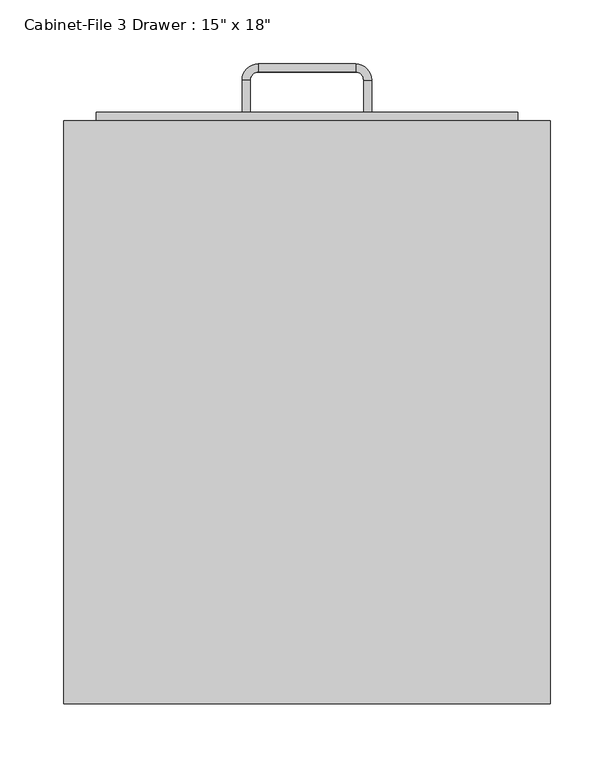
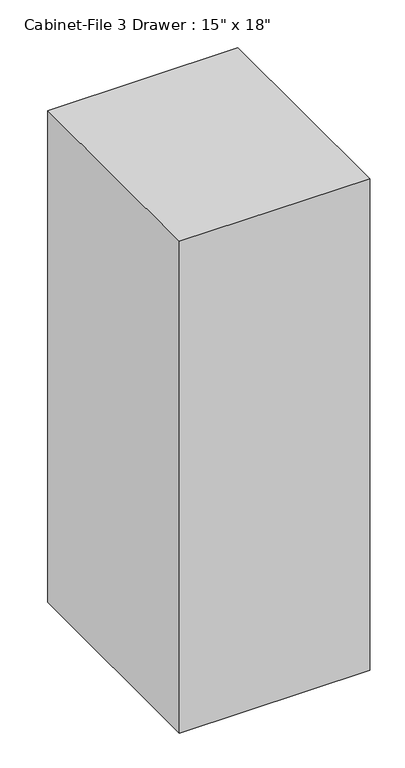
"""IFC4 building model written with IfcOpenShell, lengths in millimetres: furniture geometry."""

from ifc_helpers import new_model, si_unit, frame, origin, origin_with_axes, place, context, project, spatial, polyline, circle_curve, outline, extrude, source, transform, mapped, element, save
from ifc_brep_helpers import plane_surface, cylinder_surface, revolved_surface, advanced_brep


def furniture_48aa8ab9(model_context):
    return source(origin(), model_context, "Body", "SolidModel", [
        extrude(outline(polyline([(62.603553, -86.4656999), (-318.396447, -86.4656999), (-318.396447, 370.7343001), (62.603553, 370.7343001), (62.603553, -86.4656999)])), origin_with_axes(), (0.0, 0.0, 1.0), 1041.4),
        extrude(outline(polyline([(37.203553, 377.0843001), (37.203553, 370.7343001), (-292.996447, 370.7343001), (-292.996447, 377.0843001), (37.203553, 377.0843001)])), frame((0.0, 0.0, 736.6), z_axis=(0.0, 0.0, 1.0), x_axis=(1.0, 0.0, 0.0)), (0.0, 0.0, 1.0), 279.4),
        extrude(outline(polyline([(37.203553, 377.0843001), (37.203553, 370.7343001), (-292.996447, 370.7343001), (-292.996447, 377.0843001), (37.203553, 377.0843001)])), frame((0.0, 0.0, 431.8), z_axis=(0.0, 0.0, 1.0), x_axis=(1.0, 0.0, 0.0)), (0.0, 0.0, 1.0), 279.4),
        extrude(outline(polyline([(37.203553, 377.0843001), (37.203553, 370.7343001), (-292.996447, 370.7343001), (-292.996447, 377.0843001), (37.203553, 377.0843001)])), frame((0.0, 0.0, 127.0), z_axis=(0.0, 0.0, 1.0), x_axis=(1.0, 0.0, 0.0)), (0.0, 0.0, 1.0), 279.4),
        advanced_brep(
        [(-172.346447, 377.0843001, 203.2), (-172.346447, 377.0843001, 215.9), (-178.696447, 377.0843001, 215.9), (-178.696447, 377.0843001, 203.2), (-178.696447, 402.4843001, 203.2), (-172.346447, 402.4843001, 203.2), (-178.696447, 402.4843001, 215.9), (-172.346447, 402.4843001, 215.9), (-165.996447, 415.1843001, 203.2), (-165.996447, 408.8343001, 203.2), (-165.996447, 415.1843001, 215.9), (-165.996447, 408.8343001, 215.9), (-89.796447, 415.1843001, 203.2), (-89.796447, 408.8343001, 203.2), (-89.796447, 415.1843001, 215.9), (-89.796447, 408.8343001, 215.9), (-77.096447, 402.4843001, 203.2), (-83.446447, 402.4843001, 203.2), (-77.096447, 402.4843001, 215.9), (-83.446447, 402.4843001, 215.9), (-83.446447, 377.0843001, 203.2), (-77.096447, 377.0843001, 203.2), (-77.096447, 377.0843001, 215.9), (-83.446447, 377.0843001, 215.9)],
        [
            (0, 1),
            (1, 2),
            (2, 3),
            (3, 0),
            (3, 4),
            (4, 5),
            (5, 0),
            (2, 6),
            (6, 4),
            (1, 7),
            (7, 6),
            (5, 7),
            (8, 9),
            (9, 5, circle_curve(frame((-165.996447, 402.4843001, 203.2), z_axis=(0.0, 0.0, 1.0), x_axis=(-1.0, 0.0, 0.0)), 6.35)),
            (4, 8, circle_curve(frame((-165.996447, 402.4843001, 203.2), z_axis=(0.0, 0.0, -1.0), x_axis=(-1.0, 0.0, 0.0)), 12.7)),
            (10, 8),
            (6, 10, circle_curve(frame((-165.996447, 402.4843001, 215.9), z_axis=(0.0, 0.0, -1.0), x_axis=(-1.0, 0.0, 0.0)), 12.7)),
            (11, 10),
            (7, 11, circle_curve(frame((-165.996447, 402.4843001, 215.9), z_axis=(0.0, 0.0, -1.0), x_axis=(-1.0, 0.0, 0.0)), 6.35)),
            (9, 11),
            (8, 12),
            (12, 13),
            (13, 9),
            (10, 14),
            (14, 12),
            (11, 15),
            (15, 14),
            (13, 15),
            (16, 17),
            (17, 13, circle_curve(frame((-89.796447, 402.4843001, 203.2), z_axis=(0.0, 0.0, 1.0), x_axis=(0.0, 1.0, 0.0)), 6.35)),
            (12, 16, circle_curve(frame((-89.796447, 402.4843001, 203.2), z_axis=(0.0, 0.0, -1.0), x_axis=(0.0, 1.0, 0.0)), 12.7)),
            (18, 16),
            (14, 18, circle_curve(frame((-89.796447, 402.4843001, 215.9), z_axis=(0.0, 0.0, -1.0), x_axis=(0.0, 1.0, 0.0)), 12.7)),
            (19, 18),
            (15, 19, circle_curve(frame((-89.796447, 402.4843001, 215.9), z_axis=(0.0, 0.0, -1.0), x_axis=(0.0, 1.0, 0.0)), 6.35)),
            (17, 19),
            (20, 21),
            (21, 22),
            (22, 23),
            (23, 20),
            (16, 21),
            (20, 17),
            (18, 22),
            (19, 23),
        ],
        [
            plane_surface(frame((-978.8216451, 377.0843001, 0.0), z_axis=(0.0, -1.0, 0.0), x_axis=(0.0, 0.0, -1.0))),
            plane_surface(frame((-172.346447, 377.0843001, 203.2), z_axis=(0.0, 0.0, -1.0), x_axis=(0.0, 1.0, 0.0))),
            plane_surface(frame((-178.696447, 377.0843001, 203.2), z_axis=(-1.0, 0.0, 0.0), x_axis=(0.0, 1.0, 0.0))),
            plane_surface(frame((-178.696447, 377.0843001, 215.9), z_axis=(0.0, 0.0, 1.0), x_axis=(0.0, 1.0, 0.0))),
            plane_surface(frame((-172.346447, 377.0843001, 215.9), z_axis=(1.0, 0.0, 0.0), x_axis=(0.0, 1.0, 0.0))),
            plane_surface(frame((-165.996447, 402.4843001, 203.2), z_axis=(0.0, 0.0, -1.0), x_axis=(-1.0, 0.0, 0.0))),
            cylinder_surface(frame((-165.996447, 402.4843001, 0.0), z_axis=(0.0, 0.0, 1.0), x_axis=(-1.0, 0.0, 0.0)), 12.7),
            plane_surface(frame((-165.996447, 402.4843001, 215.9), z_axis=(0.0, 0.0, 1.0), x_axis=(-1.0, 0.0, 0.0))),
            revolved_surface(polyline([(-172.34644699999998, 402.4843001, 215.9), (-172.34644699999998, 402.4843001, 203.2)]), (-165.996447, 402.4843001, 0.0), (0.0, 0.0, 1.0)),
            plane_surface(frame((-165.996447, 408.8343001, 203.2), z_axis=(0.0, 0.0, -1.0), x_axis=(1.0, 0.0, 0.0))),
            plane_surface(frame((-165.996447, 415.1843001, 203.2), z_axis=(0.0, 1.0, 0.0), x_axis=(1.0, 0.0, 0.0))),
            plane_surface(frame((-165.996447, 415.1843001, 215.9), z_axis=(0.0, 0.0, 1.0), x_axis=(1.0, 0.0, 0.0))),
            plane_surface(frame((-165.996447, 408.8343001, 215.9), z_axis=(0.0, -1.0, 0.0), x_axis=(1.0, 0.0, 0.0))),
            plane_surface(frame((-89.796447, 402.4843001, 203.2), z_axis=(0.0, 0.0, -1.0), x_axis=(0.0, 1.0, 0.0))),
            cylinder_surface(frame((-89.796447, 402.4843001, 0.0), z_axis=(0.0, 0.0, 1.0), x_axis=(0.0, 1.0, 0.0)), 12.7),
            plane_surface(frame((-89.796447, 402.4843001, 215.9), z_axis=(0.0, 0.0, 1.0), x_axis=(0.0, 1.0, 0.0))),
            revolved_surface(polyline([(-89.796447, 408.8343001, 215.9), (-89.796447, 408.8343001, 203.2)]), (-89.796447, 402.4843001, 0.0), (0.0, 0.0, 1.0)),
            plane_surface(frame((-877.2216451, 377.0843001, 0.0), z_axis=(0.0, -1.0, 0.0), x_axis=(0.0, 0.0, 1.0))),
            plane_surface(frame((-83.446447, 402.4843001, 203.2), z_axis=(0.0, 0.0, -1.0), x_axis=(0.0, -1.0, 0.0))),
            plane_surface(frame((-77.096447, 402.4843001, 203.2), z_axis=(1.0, 0.0, 0.0), x_axis=(0.0, -1.0, 0.0))),
            plane_surface(frame((-77.096447, 402.4843001, 215.9), z_axis=(0.0, 0.0, 1.0), x_axis=(0.0, -1.0, 0.0))),
            plane_surface(frame((-83.446447, 402.4843001, 215.9), z_axis=(-1.0, 0.0, 0.0), x_axis=(0.0, -1.0, 0.0))),
        ],
        [
            (0, [[1, 2, 3, 4]]),
            (1, [[5, 6, 7, -4]]),
            (2, [[8, 9, -5, -3]]),
            (3, [[10, 11, -8, -2]]),
            (4, [[-7, 12, -10, -1]]),
            (5, [[13, 14, -6, 15]]),
            (6, [[16, -15, -9, 17]]),
            (7, [[18, -17, -11, 19]]),
            (8, [[20, -19, -12, -14]]),
            (9, [[21, 22, 23, -13]]),
            (10, [[24, 25, -21, -16]]),
            (11, [[26, 27, -24, -18]]),
            (12, [[-23, 28, -26, -20]]),
            (13, [[29, 30, -22, 31]]),
            (14, [[32, -31, -25, 33]]),
            (15, [[34, -33, -27, 35]]),
            (16, [[36, -35, -28, -30]]),
            (17, [[37, 38, 39, 40]]),
            (18, [[41, -37, 42, -29]]),
            (19, [[43, -38, -41, -32]]),
            (20, [[44, -39, -43, -34]]),
            (21, [[-42, -40, -44, -36]]),
        ],
    ),
        advanced_brep(
        [(-172.346447, 377.0843001, 482.6), (-172.346447, 377.0843001, 495.3), (-178.696447, 377.0843001, 495.3), (-178.696447, 377.0843001, 482.6), (-178.696447, 402.4843001, 482.6), (-172.346447, 402.4843001, 482.6), (-178.696447, 402.4843001, 495.3), (-172.346447, 402.4843001, 495.3), (-165.996447, 415.1843001, 482.6), (-165.996447, 408.8343001, 482.6), (-165.996447, 415.1843001, 495.3), (-165.996447, 408.8343001, 495.3), (-89.796447, 415.1843001, 482.6), (-89.796447, 408.8343001, 482.6), (-89.796447, 415.1843001, 495.3), (-89.796447, 408.8343001, 495.3), (-77.096447, 402.4843001, 482.6), (-83.446447, 402.4843001, 482.6), (-77.096447, 402.4843001, 495.3), (-83.446447, 402.4843001, 495.3), (-83.446447, 377.0843001, 482.6), (-77.096447, 377.0843001, 482.6), (-77.096447, 377.0843001, 495.3), (-83.446447, 377.0843001, 495.3)],
        [
            (0, 1),
            (1, 2),
            (2, 3),
            (3, 0),
            (3, 4),
            (4, 5),
            (5, 0),
            (2, 6),
            (6, 4),
            (1, 7),
            (7, 6),
            (5, 7),
            (8, 9),
            (9, 5, circle_curve(frame((-165.996447, 402.4843001, 482.6), z_axis=(0.0, 0.0, 1.0), x_axis=(-1.0, 0.0, 0.0)), 6.35)),
            (4, 8, circle_curve(frame((-165.996447, 402.4843001, 482.6), z_axis=(0.0, 0.0, -1.0), x_axis=(-1.0, 0.0, 0.0)), 12.7)),
            (10, 8),
            (6, 10, circle_curve(frame((-165.996447, 402.4843001, 495.3), z_axis=(0.0, 0.0, -1.0), x_axis=(-1.0, 0.0, 0.0)), 12.7)),
            (11, 10),
            (7, 11, circle_curve(frame((-165.996447, 402.4843001, 495.3), z_axis=(0.0, 0.0, -1.0), x_axis=(-1.0, 0.0, 0.0)), 6.35)),
            (9, 11),
            (8, 12),
            (12, 13),
            (13, 9),
            (10, 14),
            (14, 12),
            (11, 15),
            (15, 14),
            (13, 15),
            (16, 17),
            (17, 13, circle_curve(frame((-89.796447, 402.4843001, 482.6), z_axis=(0.0, 0.0, 1.0), x_axis=(0.0, 1.0, 0.0)), 6.35)),
            (12, 16, circle_curve(frame((-89.796447, 402.4843001, 482.6), z_axis=(0.0, 0.0, -1.0), x_axis=(0.0, 1.0, 0.0)), 12.7)),
            (18, 16),
            (14, 18, circle_curve(frame((-89.796447, 402.4843001, 495.3), z_axis=(0.0, 0.0, -1.0), x_axis=(0.0, 1.0, 0.0)), 12.7)),
            (19, 18),
            (15, 19, circle_curve(frame((-89.796447, 402.4843001, 495.3), z_axis=(0.0, 0.0, -1.0), x_axis=(0.0, 1.0, 0.0)), 6.35)),
            (17, 19),
            (20, 21),
            (21, 22),
            (22, 23),
            (23, 20),
            (16, 21),
            (20, 17),
            (18, 22),
            (19, 23),
        ],
        [
            plane_surface(frame((-978.8216451, 377.0843001, 0.0), z_axis=(0.0, -1.0, 0.0), x_axis=(0.0, 0.0, -1.0))),
            plane_surface(frame((-172.346447, 377.0843001, 482.6), z_axis=(0.0, 0.0, -1.0), x_axis=(0.0, 1.0, 0.0))),
            plane_surface(frame((-178.696447, 377.0843001, 482.6), z_axis=(-1.0, 0.0, 0.0), x_axis=(0.0, 1.0, 0.0))),
            plane_surface(frame((-178.696447, 377.0843001, 495.3), z_axis=(0.0, 0.0, 1.0), x_axis=(0.0, 1.0, 0.0))),
            plane_surface(frame((-172.346447, 377.0843001, 495.3), z_axis=(1.0, 0.0, 0.0), x_axis=(0.0, 1.0, 0.0))),
            plane_surface(frame((-165.996447, 402.4843001, 482.6), z_axis=(0.0, 0.0, -1.0), x_axis=(-1.0, 0.0, 0.0))),
            cylinder_surface(frame((-165.996447, 402.4843001, 0.0), z_axis=(0.0, 0.0, 1.0), x_axis=(-1.0, 0.0, 0.0)), 12.7),
            plane_surface(frame((-165.996447, 402.4843001, 495.3), z_axis=(0.0, 0.0, 1.0), x_axis=(-1.0, 0.0, 0.0))),
            revolved_surface(polyline([(-172.34644699999998, 402.4843001, 495.3), (-172.34644699999998, 402.4843001, 482.6)]), (-165.996447, 402.4843001, 0.0), (0.0, 0.0, 1.0)),
            plane_surface(frame((-165.996447, 408.8343001, 482.6), z_axis=(0.0, 0.0, -1.0), x_axis=(1.0, 0.0, 0.0))),
            plane_surface(frame((-165.996447, 415.1843001, 482.6), z_axis=(0.0, 1.0, 0.0), x_axis=(1.0, 0.0, 0.0))),
            plane_surface(frame((-165.996447, 415.1843001, 495.3), z_axis=(0.0, 0.0, 1.0), x_axis=(1.0, 0.0, 0.0))),
            plane_surface(frame((-165.996447, 408.8343001, 495.3), z_axis=(0.0, -1.0, 0.0), x_axis=(1.0, 0.0, 0.0))),
            plane_surface(frame((-89.796447, 402.4843001, 482.6), z_axis=(0.0, 0.0, -1.0), x_axis=(0.0, 1.0, 0.0))),
            cylinder_surface(frame((-89.796447, 402.4843001, 0.0), z_axis=(0.0, 0.0, 1.0), x_axis=(0.0, 1.0, 0.0)), 12.7),
            plane_surface(frame((-89.796447, 402.4843001, 495.3), z_axis=(0.0, 0.0, 1.0), x_axis=(0.0, 1.0, 0.0))),
            revolved_surface(polyline([(-89.796447, 408.8343001, 495.3), (-89.796447, 408.8343001, 482.6)]), (-89.796447, 402.4843001, 0.0), (0.0, 0.0, 1.0)),
            plane_surface(frame((-877.2216451, 377.0843001, 0.0), z_axis=(0.0, -1.0, 0.0), x_axis=(0.0, 0.0, 1.0))),
            plane_surface(frame((-83.446447, 402.4843001, 482.6), z_axis=(0.0, 0.0, -1.0), x_axis=(0.0, -1.0, 0.0))),
            plane_surface(frame((-77.096447, 402.4843001, 482.6), z_axis=(1.0, 0.0, 0.0), x_axis=(0.0, -1.0, 0.0))),
            plane_surface(frame((-77.096447, 402.4843001, 495.3), z_axis=(0.0, 0.0, 1.0), x_axis=(0.0, -1.0, 0.0))),
            plane_surface(frame((-83.446447, 402.4843001, 495.3), z_axis=(-1.0, 0.0, 0.0), x_axis=(0.0, -1.0, 0.0))),
        ],
        [
            (0, [[1, 2, 3, 4]]),
            (1, [[5, 6, 7, -4]]),
            (2, [[8, 9, -5, -3]]),
            (3, [[10, 11, -8, -2]]),
            (4, [[-7, 12, -10, -1]]),
            (5, [[13, 14, -6, 15]]),
            (6, [[16, -15, -9, 17]]),
            (7, [[18, -17, -11, 19]]),
            (8, [[20, -19, -12, -14]]),
            (9, [[21, 22, 23, -13]]),
            (10, [[24, 25, -21, -16]]),
            (11, [[26, 27, -24, -18]]),
            (12, [[-23, 28, -26, -20]]),
            (13, [[29, 30, -22, 31]]),
            (14, [[32, -31, -25, 33]]),
            (15, [[34, -33, -27, 35]]),
            (16, [[36, -35, -28, -30]]),
            (17, [[37, 38, 39, 40]]),
            (18, [[41, -37, 42, -29]]),
            (19, [[43, -38, -41, -32]]),
            (20, [[44, -39, -43, -34]]),
            (21, [[-42, -40, -44, -36]]),
        ],
    ),
        advanced_brep(
        [(-172.346447, 377.0843001, 787.4), (-172.346447, 377.0843001, 800.1), (-178.696447, 377.0843001, 800.1), (-178.696447, 377.0843001, 787.4), (-178.696447, 402.4843001, 787.4), (-172.346447, 402.4843001, 787.4), (-178.696447, 402.4843001, 800.1), (-172.346447, 402.4843001, 800.1), (-165.996447, 415.1843001, 787.4), (-165.996447, 408.8343001, 787.4), (-165.996447, 415.1843001, 800.1), (-165.996447, 408.8343001, 800.1), (-89.796447, 415.1843001, 787.4), (-89.796447, 408.8343001, 787.4), (-89.796447, 415.1843001, 800.1), (-89.796447, 408.8343001, 800.1), (-77.096447, 402.4843001, 787.4), (-83.446447, 402.4843001, 787.4), (-77.096447, 402.4843001, 800.1), (-83.446447, 402.4843001, 800.1), (-83.446447, 377.0843001, 787.4), (-77.096447, 377.0843001, 787.4), (-77.096447, 377.0843001, 800.1), (-83.446447, 377.0843001, 800.1)],
        [
            (0, 1),
            (1, 2),
            (2, 3),
            (3, 0),
            (3, 4),
            (4, 5),
            (5, 0),
            (2, 6),
            (6, 4),
            (1, 7),
            (7, 6),
            (5, 7),
            (8, 9),
            (9, 5, circle_curve(frame((-165.996447, 402.4843001, 787.4), z_axis=(0.0, 0.0, 1.0), x_axis=(-1.0, 0.0, 0.0)), 6.35)),
            (4, 8, circle_curve(frame((-165.996447, 402.4843001, 787.4), z_axis=(0.0, 0.0, -1.0), x_axis=(-1.0, 0.0, 0.0)), 12.7)),
            (10, 8),
            (6, 10, circle_curve(frame((-165.996447, 402.4843001, 800.1), z_axis=(0.0, 0.0, -1.0), x_axis=(-1.0, 0.0, 0.0)), 12.7)),
            (11, 10),
            (7, 11, circle_curve(frame((-165.996447, 402.4843001, 800.1), z_axis=(0.0, 0.0, -1.0), x_axis=(-1.0, 0.0, 0.0)), 6.35)),
            (9, 11),
            (8, 12),
            (12, 13),
            (13, 9),
            (10, 14),
            (14, 12),
            (11, 15),
            (15, 14),
            (13, 15),
            (16, 17),
            (17, 13, circle_curve(frame((-89.796447, 402.4843001, 787.4), z_axis=(0.0, 0.0, 1.0), x_axis=(0.0, 1.0, 0.0)), 6.35)),
            (12, 16, circle_curve(frame((-89.796447, 402.4843001, 787.4), z_axis=(0.0, 0.0, -1.0), x_axis=(0.0, 1.0, 0.0)), 12.7)),
            (18, 16),
            (14, 18, circle_curve(frame((-89.796447, 402.4843001, 800.1), z_axis=(0.0, 0.0, -1.0), x_axis=(0.0, 1.0, 0.0)), 12.7)),
            (19, 18),
            (15, 19, circle_curve(frame((-89.796447, 402.4843001, 800.1), z_axis=(0.0, 0.0, -1.0), x_axis=(0.0, 1.0, 0.0)), 6.35)),
            (17, 19),
            (20, 21),
            (21, 22),
            (22, 23),
            (23, 20),
            (16, 21),
            (20, 17),
            (18, 22),
            (19, 23),
        ],
        [
            plane_surface(frame((-978.8216451, 377.0843001, 0.0), z_axis=(0.0, -1.0, 0.0), x_axis=(0.0, 0.0, -1.0))),
            plane_surface(frame((-172.346447, 377.0843001, 787.4), z_axis=(0.0, 0.0, -1.0), x_axis=(0.0, 1.0, 0.0))),
            plane_surface(frame((-178.696447, 377.0843001, 787.4), z_axis=(-1.0, 0.0, 0.0), x_axis=(0.0, 1.0, 0.0))),
            plane_surface(frame((-178.696447, 377.0843001, 800.1), z_axis=(0.0, 0.0, 1.0), x_axis=(0.0, 1.0, 0.0))),
            plane_surface(frame((-172.346447, 377.0843001, 800.1), z_axis=(1.0, 0.0, 0.0), x_axis=(0.0, 1.0, 0.0))),
            plane_surface(frame((-165.996447, 402.4843001, 787.4), z_axis=(0.0, 0.0, -1.0), x_axis=(-1.0, 0.0, 0.0))),
            cylinder_surface(frame((-165.996447, 402.4843001, 0.0), z_axis=(0.0, 0.0, 1.0), x_axis=(-1.0, 0.0, 0.0)), 12.7),
            plane_surface(frame((-165.996447, 402.4843001, 800.1), z_axis=(0.0, 0.0, 1.0), x_axis=(-1.0, 0.0, 0.0))),
            revolved_surface(polyline([(-172.34644699999998, 402.4843001, 800.1), (-172.34644699999998, 402.4843001, 787.4)]), (-165.996447, 402.4843001, 0.0), (0.0, 0.0, 1.0)),
            plane_surface(frame((-165.996447, 408.8343001, 787.4), z_axis=(0.0, 0.0, -1.0), x_axis=(1.0, 0.0, 0.0))),
            plane_surface(frame((-165.996447, 415.1843001, 787.4), z_axis=(0.0, 1.0, 0.0), x_axis=(1.0, 0.0, 0.0))),
            plane_surface(frame((-165.996447, 415.1843001, 800.1), z_axis=(0.0, 0.0, 1.0), x_axis=(1.0, 0.0, 0.0))),
            plane_surface(frame((-165.996447, 408.8343001, 800.1), z_axis=(0.0, -1.0, 0.0), x_axis=(1.0, 0.0, 0.0))),
            plane_surface(frame((-89.796447, 402.4843001, 787.4), z_axis=(0.0, 0.0, -1.0), x_axis=(0.0, 1.0, 0.0))),
            cylinder_surface(frame((-89.796447, 402.4843001, 0.0), z_axis=(0.0, 0.0, 1.0), x_axis=(0.0, 1.0, 0.0)), 12.7),
            plane_surface(frame((-89.796447, 402.4843001, 800.1), z_axis=(0.0, 0.0, 1.0), x_axis=(0.0, 1.0, 0.0))),
            revolved_surface(polyline([(-89.796447, 408.8343001, 800.1), (-89.796447, 408.8343001, 787.4)]), (-89.796447, 402.4843001, 0.0), (0.0, 0.0, 1.0)),
            plane_surface(frame((-877.2216451, 377.0843001, 0.0), z_axis=(0.0, -1.0, 0.0), x_axis=(0.0, 0.0, 1.0))),
            plane_surface(frame((-83.446447, 402.4843001, 787.4), z_axis=(0.0, 0.0, -1.0), x_axis=(0.0, -1.0, 0.0))),
            plane_surface(frame((-77.096447, 402.4843001, 787.4), z_axis=(1.0, 0.0, 0.0), x_axis=(0.0, -1.0, 0.0))),
            plane_surface(frame((-77.096447, 402.4843001, 800.1), z_axis=(0.0, 0.0, 1.0), x_axis=(0.0, -1.0, 0.0))),
            plane_surface(frame((-83.446447, 402.4843001, 800.1), z_axis=(-1.0, 0.0, 0.0), x_axis=(0.0, -1.0, 0.0))),
        ],
        [
            (0, [[1, 2, 3, 4]]),
            (1, [[5, 6, 7, -4]]),
            (2, [[8, 9, -5, -3]]),
            (3, [[10, 11, -8, -2]]),
            (4, [[-7, 12, -10, -1]]),
            (5, [[13, 14, -6, 15]]),
            (6, [[16, -15, -9, 17]]),
            (7, [[18, -17, -11, 19]]),
            (8, [[20, -19, -12, -14]]),
            (9, [[21, 22, 23, -13]]),
            (10, [[24, 25, -21, -16]]),
            (11, [[26, 27, -24, -18]]),
            (12, [[-23, 28, -26, -20]]),
            (13, [[29, 30, -22, 31]]),
            (14, [[32, -31, -25, 33]]),
            (15, [[34, -33, -27, 35]]),
            (16, [[36, -35, -28, -30]]),
            (17, [[37, 38, 39, 40]]),
            (18, [[41, -37, 42, -29]]),
            (19, [[43, -38, -41, -32]]),
            (20, [[44, -39, -43, -34]]),
            (21, [[-42, -40, -44, -36]]),
        ],
    ),
    ])


if __name__ == "__main__":
    model = new_model("IFC4")
    model_context = context("Model", 3, world=origin())
    ifc_project = project(units=[si_unit("LENGTHUNIT", "METRE", prefix="MILLI")], contexts=[model_context])
    site = spatial("IfcSite", under=ifc_project)
    building = spatial("IfcBuilding", under=site)
    placement = place(None, origin())
    furniture_shape = furniture_48aa8ab9(model_context)
    element("IfcFurniture", 1, ObjectType="Cabinet-File 3 Drawer : 15\" x 18\"", at=placement, inside=building, context=model_context, shape_type="MappedRepresentation", body=[
        mapped(furniture_shape, transform((0.0, 0.0, 0.0), x_axis=(1.0, 0.0, 0.0), y_axis=(0.0, 1.0, 0.0), z_axis=(0.0, 0.0, 1.0))),
    ])
    save(model, "model.ifc")

# Revit data of these elements
# Type "Cabinet-File 3 Drawer : 15\" x 18\""
#   Assembly Code = "E2020200"
#   Depth = 1' - 6"
#   Height = 3' - 5"
#   Width = 1' - 3"
#   Cabinet Material = Steel, Paint Finish, Ivory, Glossy
#   Handle Material = Steel, Chrome Plated
#   Default Elevation = 0
# Element 1 (IfcFurniture, "Cabinet-File 3 Drawer : 15\" x 18\"")
#   Materials on its faces: "Steel, Chrome Plated", "Steel, Paint Finish, Ivory, Glossy"
# Materials
#   "Steel, Paint Finish, Ivory, Glossy": class "Metal", colour RGB 247 247 239, transparency 0, Description = "Steel, paint finish, ivory, glossy", Cost = 0
#   "Steel, Chrome Plated": class "Metal", colour RGB 17 17 17, transparency 0, Description = "Chromiuim plated steel", Cost = 0
